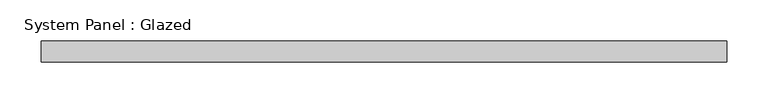
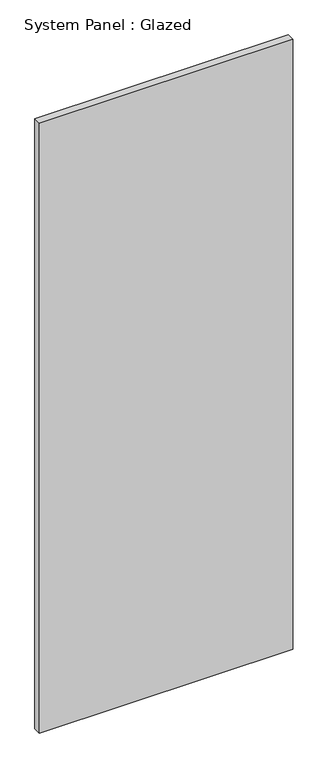
"""IFC4 building model written with IfcOpenShell, lengths in millimetres: plate geometry, System Panel : Glazed."""

from ifc_helpers import new_model, si_unit, origin, origin_with_axes, place, context, project, spatial, polyline, outline, extrude, source, transform, mapped, element, save


def system_panel_glazed_1b99a4e4(model_context):
    return source(origin(), model_context, "Body", "SweptSolid", [
        extrude(outline(polyline([(414.0389939, 19.05), (-414.0389939, 19.05), (-414.0389939, 44.45), (414.0389939, 44.45), (414.0389939, 19.05)])), origin_with_axes(), (0.0, 0.0, 1.0), 2108.2),
    ])


if __name__ == "__main__":
    model = new_model("IFC4")
    model_context = context("Model", 3, world=origin())
    ifc_project = project(units=[si_unit("LENGTHUNIT", "METRE", prefix="MILLI")], contexts=[model_context])
    site = spatial("IfcSite", under=ifc_project)
    building = spatial("IfcBuilding", under=site)
    placement = place(None, origin())
    system_panel_glazed_shape = system_panel_glazed_1b99a4e4(model_context)
    element("IfcPlate", 1, ObjectType="System Panel : Glazed", at=placement, inside=building, context=model_context, shape_type="MappedRepresentation", body=[
        mapped(system_panel_glazed_shape, transform((0.0, 0.0, 0.0), x_axis=(1.0, 0.0, 0.0), y_axis=(0.0, 1.0, 0.0), z_axis=(0.0, 0.0, 1.0))),
    ])
    save(model, "model.ifc")

# Revit data of these elements
# Type "System Panel : Glazed"
#   Construction Type Id = "GSP4R"
#   Analytic Construction = "1/8 in Pilkington single glazing"
#   Visual Light Transmittance = 0.9
#   Solar Heat Gain Coefficient = 0.86
#   Heat Transfer Coefficient (U) = 1.18115 BTU/(h·ft²·°F)
#   Define Thermal Properties by = 1
# Element 1 (IfcPlate, "System Panel : Glazed")
#   Materials on its faces: "Glass"
# Materials
#   "Glass": class "Glass", colour RGB 0 128 192, transparency 0.75, Description = "Soda Lime Glass", Cost = 0
